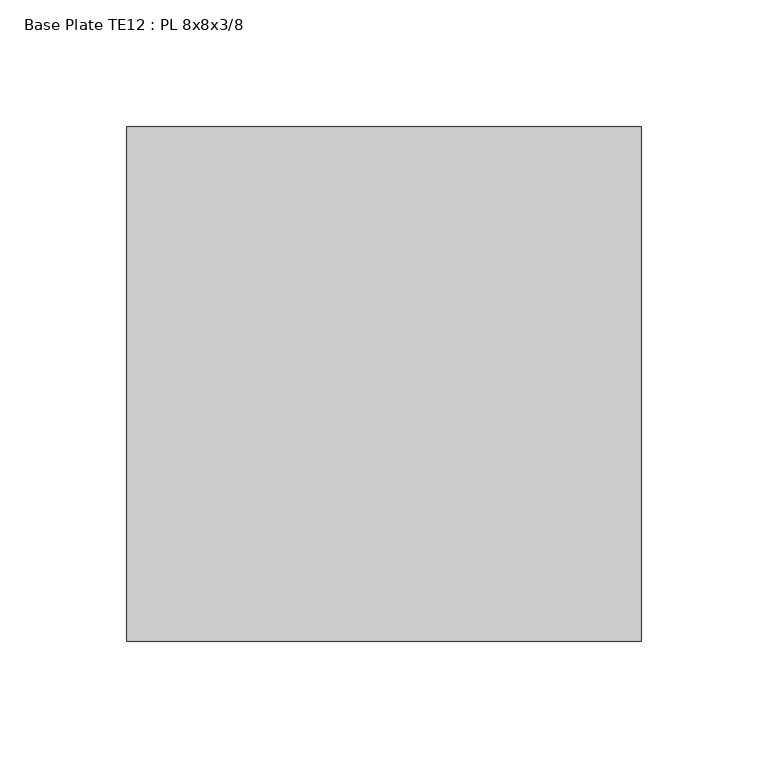
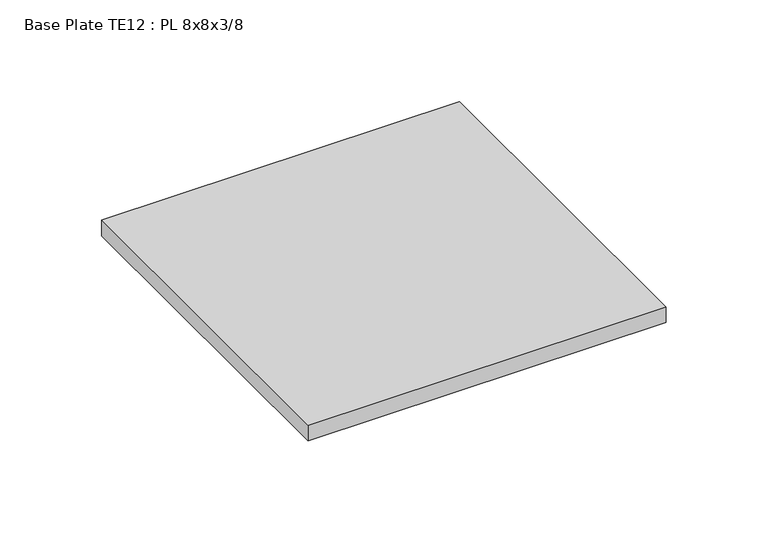
"""IFC4 building model written with IfcOpenShell, lengths in millimetres: proxy geometry, Base Plate TE12 : PL 8x8x3/8."""

from ifc_helpers import new_model, si_unit, frame, origin, place, context, project, spatial, polyline, outline, extrude, source, transform, mapped, element, save


def base_plate_te12_pl_8x8x3_8_af136eb6(model_context):
    return source(origin(), model_context, "Body", "SweptSolid", [
        extrude(outline(polyline([(590318.6599233, -535103.1413841), (590318.6599233, -535306.3413841), (590115.4599233, -535306.3413841), (590115.4599233, -535103.1413841), (590318.6599233, -535103.1413841)])), frame((0.0, 0.0, 19.05), z_axis=(0.0, 0.0, 1.0), x_axis=(1.0, 0.0, 0.0)), (0.0, 0.0, 1.0), 9.525),
    ])


if __name__ == "__main__":
    model = new_model("IFC4")
    model_context = context("Model", 3, world=origin())
    ifc_project = project(units=[si_unit("LENGTHUNIT", "METRE", prefix="MILLI")], contexts=[model_context])
    site = spatial("IfcSite", under=ifc_project)
    building = spatial("IfcBuilding", under=site)
    placement = place(None, origin())
    base_plate_te12_pl_8x8x3_8_shape = base_plate_te12_pl_8x8x3_8_af136eb6(model_context)
    element("IfcBuildingElementProxy", 1, Name="Base Plate TE12 : PL 8x8x3/8", ObjectType="Base Plate TE12 : PL 8x8x3/8", at=placement, inside=building, context=model_context, shape_type="MappedRepresentation", body=[
        mapped(base_plate_te12_pl_8x8x3_8_shape, transform((0.0, 0.0, 0.0), x_axis=(1.0, 0.0, 0.0), y_axis=(0.0, 1.0, 0.0), z_axis=(0.0, 0.0, 1.0))),
    ])
    save(model, "model.ifc")

# Revit data of these elements
# Element 1 (IfcBuildingElementProxy, "Base Plate TE12 : PL 8x8x3/8")
#   Materials on its faces: "GALV. STL BASE PLATE"
# Materials
#   "GALV. STL BASE PLATE": class "Generic", colour RGB 211 211 207, transparency 0, Cost = 0
